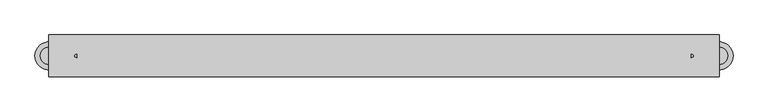
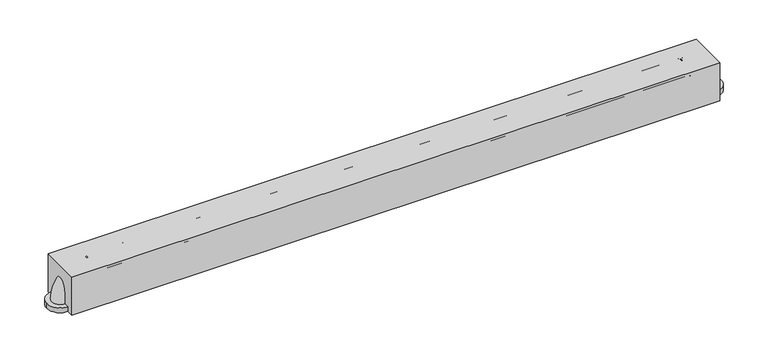
"""IFC4 building model written with IfcOpenShell, lengths in millimetres: proxy geometry, A5109 - Grab Bar, 1.25 in Dia, SS, 2 Wall, W-C Accessible : A5109 - Grab Bar, 1.25 in Dia, SS, 2 Wall, W-C Accessible."""

from ifc_helpers import new_model, si_unit, point, frame, frame_2d, origin, origin_with_axes, place, context, project, spatial, polyline, circle_curve, ellipse_curve, trimmed, segment, composite_curve, outline, extrude, source, transform, mapped, element, save
from ifc_brep_helpers import plane_surface, revolved_surface, advanced_brep


def specialty_equipment_c5804665(model_context):
    return source(origin(), model_context, "Body", "SolidModel", [
        advanced_brep(
        [(558.8, 15.875, 60.325), (558.8, -15.875, 60.325), (609.6, 15.875, 9.525), (609.6, -15.875, 9.525)],
        [
            (0, 1, circle_curve(frame((558.8, 0.0, 60.325), z_axis=(-1.0, 0.0, 0.0), x_axis=(0.0, -1.0, 0.0)), 15.875)),
            (1, 0, circle_curve(frame((558.8, 0.0, 60.325), z_axis=(-1.0, 0.0, 0.0), x_axis=(0.0, -1.0, 0.0)), 15.875)),
            (2, 3, circle_curve(frame((609.6, 0.0, 9.525), z_axis=(0.0, 0.0, -1.0), x_axis=(0.0, -1.0, 0.0)), 15.875)),
            (3, 2, circle_curve(frame((609.6, 0.0, 9.525), z_axis=(0.0, 0.0, -1.0), x_axis=(0.0, -1.0, 0.0)), 15.875)),
            (2, 0, circle_curve(frame((558.8, 15.875, 9.525), z_axis=(0.0, -1.0, 0.0), x_axis=(0.0, 0.0, 1.0)), 50.8)),
            (1, 3, circle_curve(frame((558.8, -15.875, 9.525), z_axis=(0.0, 1.0, 0.0), x_axis=(0.0, 0.0, 1.0)), 50.8)),
        ],
        [
            plane_surface(frame((558.8, 0.0, 60.325), z_axis=(-1.0, 0.0, 0.0), x_axis=(0.0, -1.0, 0.0))),
            plane_surface(frame((609.6, 0.0, 9.525), z_axis=(0.0, 0.0, -1.0), x_axis=(0.0, -1.0, 0.0))),
            revolved_surface(trimmed(ellipse_curve(frame((558.8, 0.0, 60.325), z_axis=(1.0, 0.0, 0.0), x_axis=(0.0, -1.0, 0.0)), 15.875, 15.875), [point((558.8, 15.875, 60.325))], [point((558.8, -15.875, 60.325))], True, "CARTESIAN"), (558.8, 0.0, 9.525), (0.0, -1.0, 0.0)),
            revolved_surface(trimmed(ellipse_curve(frame((558.8, 0.0, 60.325), z_axis=(1.0, 0.0, 0.0), x_axis=(0.0, -1.0, 0.0)), 15.875, 15.875), [point((558.8, -15.875, 60.325))], [point((558.8, 15.875, 60.325))], True, "CARTESIAN"), (558.8, 0.0, 9.525), (0.0, -1.0, 0.0)),
        ],
        [
            (0, [[1, 2]]),
            (1, [[3, 4]]),
            (2, [[-3, 5, -2, 6]]),
            (3, [[-4, -6, -1, -5]]),
        ],
    ),
        extrude(outline(composite_curve([segment(trimmed(circle_curve(frame_2d((609.6, 0.0)), 25.4), [point((635.0, 0.0))], [point((584.2, 0.0))], False, "CARTESIAN"), True, "CONTINUOUS"), segment(trimmed(circle_curve(frame_2d((609.6, 0.0)), 25.4), [point((584.2, 0.0))], [point((635.0, 0.0))], False, "CARTESIAN"), True, "CONTINUOUS")], self_intersect=False)), origin_with_axes(), (0.0, 0.0, 1.0), 9.525),
        advanced_brep(
        [(-558.8, 15.875, 60.325), (-558.8, -15.875, 60.325), (-609.6, 15.875, 9.525), (-609.6, -15.875, 9.525)],
        [
            (0, 1, circle_curve(frame((-558.8, 0.0, 60.325), z_axis=(1.0, 0.0, 0.0), x_axis=(0.0, -1.0, 0.0)), 15.875)),
            (1, 0, circle_curve(frame((-558.8, 0.0, 60.325), z_axis=(1.0, 0.0, 0.0), x_axis=(0.0, -1.0, 0.0)), 15.875)),
            (2, 3, circle_curve(frame((-609.6, 0.0, 9.525), z_axis=(0.0, 0.0, -1.0), x_axis=(0.0, -1.0, 0.0)), 15.875)),
            (3, 2, circle_curve(frame((-609.6, 0.0, 9.525), z_axis=(0.0, 0.0, -1.0), x_axis=(0.0, -1.0, 0.0)), 15.875)),
            (3, 1, circle_curve(frame((-558.8, -15.875, 9.525), z_axis=(0.0, 1.0, 0.0), x_axis=(0.0, 0.0, 1.0)), 50.8)),
            (0, 2, circle_curve(frame((-558.8, 15.875, 9.525), z_axis=(0.0, -1.0, 0.0), x_axis=(0.0, 0.0, 1.0)), 50.8)),
        ],
        [
            plane_surface(frame((-558.8, 0.0, 60.325), z_axis=(1.0, 0.0, 0.0), x_axis=(0.0, -1.0, 0.0))),
            plane_surface(frame((-609.6, 0.0, 9.525), z_axis=(0.0, 0.0, -1.0), x_axis=(0.0, -1.0, 0.0))),
            revolved_surface(trimmed(ellipse_curve(frame((-558.8, 0.0, 60.325), z_axis=(1.0, 0.0, 0.0), x_axis=(0.0, -1.0, 0.0)), 15.875, 15.875), [point((-558.8, 15.875, 60.325))], [point((-558.8, -15.875, 60.325))], True, "CARTESIAN"), (-558.8, 0.0, 9.525), (0.0, -1.0, 0.0)),
            revolved_surface(trimmed(ellipse_curve(frame((-558.8, 0.0, 60.325), z_axis=(1.0, 0.0, 0.0), x_axis=(0.0, -1.0, 0.0)), 15.875, 15.875), [point((-558.8, -15.875, 60.325))], [point((-558.8, 15.875, 60.325))], True, "CARTESIAN"), (-558.8, 0.0, 9.525), (0.0, -1.0, 0.0)),
        ],
        [
            (0, [[1, 2]]),
            (1, [[3, 4]]),
            (2, [[5, -1, 6, -4]]),
            (3, [[-6, -2, -5, -3]]),
        ],
    ),
        extrude(outline(composite_curve([segment(trimmed(circle_curve(frame_2d((-609.6, 0.0)), 25.4), [point((-635.0, 0.0))], [point((-584.2, 0.0))], False, "CARTESIAN"), True, "CONTINUOUS"), segment(trimmed(circle_curve(frame_2d((-609.6, 0.0)), 25.4), [point((-584.2, 0.0))], [point((-635.0, 0.0))], False, "CARTESIAN"), True, "CONTINUOUS")], self_intersect=False)), origin_with_axes(), (0.0, 0.0, 1.0), 9.525),
        extrude(outline(polyline([(609.6, -38.1), (-609.6, -38.1), (-609.6, 38.1), (609.6, 38.1), (609.6, -38.1)])), origin_with_axes(), (0.0, 0.0, 1.0), 76.2),
        extrude(outline(composite_curve([segment(trimmed(circle_curve(frame_2d((0.0, 60.325)), 15.875), [point((-15.875, 60.325))], [point((15.875, 60.325))], False, "CARTESIAN"), True, "CONTINUOUS"), segment(trimmed(circle_curve(frame_2d((0.0, 60.325)), 15.875), [point((15.875, 60.325))], [point((-15.875, 60.325))], False, "CARTESIAN"), True, "CONTINUOUS")], self_intersect=False)), frame((-558.8, 0.0, 0.0), z_axis=(1.0, 0.0, 0.0), x_axis=(0.0, 1.0, 0.0)), (0.0, 0.0, 1.0), 1117.6),
    ])


if __name__ == "__main__":
    model = new_model("IFC4")
    model_context = context("Model", 3, world=origin())
    ifc_project = project(units=[si_unit("LENGTHUNIT", "METRE", prefix="MILLI")], contexts=[model_context])
    site = spatial("IfcSite", under=ifc_project)
    building = spatial("IfcBuilding", under=site)
    placement = place(None, origin())
    specialty_equipment_shape = specialty_equipment_c5804665(model_context)
    element("IfcBuildingElementProxy", 1, Name="A5109 - Grab Bar, 1.25 in Dia, SS, 2 Wall, W-C Accessible : A5109 - Grab Bar, 1.25 in Dia, SS, 2 Wall, W-C Accessible", ObjectType="A5109 - Grab Bar, 1.25 in Dia, SS, 2 Wall, W-C Accessible : A5109 - Grab Bar, 1.25 in Dia, SS, 2 Wall, W-C Accessible", at=placement, inside=building, context=model_context, shape_type="MappedRepresentation", body=[
        mapped(specialty_equipment_shape, transform((0.0, 0.0, 0.0), x_axis=(1.0, 0.0, 0.0), y_axis=(0.0, 1.0, 0.0), z_axis=(0.0, 0.0, 1.0))),
    ])
    save(model, "model.ifc")

# Revit data of these elements
# Type "A5109 - Grab Bar, 1.25 in Dia, SS, 2 Wall, W-C Accessible : A5109 - Grab Bar, 1.25 in Dia, SS, 2 Wall, W-C Accessible"
#   Watts2 = "0"
#   Watts1 = "0"
#   Unit_Issue = "EA"
#   UTIL_6_Misc = "-"
#   UTIL_5_NonMedGas = "-"
#   UTIL_4_MiscGas = "-"
#   UTIL_3_MedGas = "-"
#   UTIL_2_Elec = "-"
#   UTIL_1_WaterDrain = "-"
#   Nomenclature = "Grab Bar, 1-1/4\" Dia., SS, 2 Wall, W/C Accessible"
#   NSN = "6530"
#   Location [instance default] = ""
#   JSN = "A5109"
#   Fund_Source_VA = "-"
#   Fund_Source_Navy = "-"
#   Fund_Source_Army = "-"
#   Fund_Source_AF = "-"
#   ELEC_Volts2 = "0"
#   ELEC_Volts1 = "0"
#   ELEC_Phase2 = "0"
#   ELEC_Phase1 = "0"
#   ELEC_HertzSwitch = "0"
#   ELEC_HertzDependent = "0"
#   ELEC_Hertz = "0"
#   ELEC_Amps2 = "0"
#   ELEC_Amps1 = "0"
#   DetailDescription = "A 1-1/4\" diameter, satin finish stainless steel, peened gripping surface, 2 wall toilet stall/ room, grab bar with concealed mounting flanges.  Snap over flanges are provided to conceal mounting screws. A selection of mounting kits and concealed anchor devices are available from the manufacturers for different types of installations. Grab bar shall comply with barrier-free accessibility guidelines for structural strength. For typical water closet applications in toilet stalls and rooms where ADA (American''s With Disabilities Act) requirements must be met."
#   CAT_VA = "A"
#   CAT_Navy = "A"
#   CAT_IHS = "-"
#   CAT_Army = "A"
#   CAT_AF = "A"
#   BTUperhour = "0"
#   Weight_IP = 7
#   Default Elevation = 2' - 9"
#   DIM_Width_IP = 4' - 9"
#   DIM_Height_IP = 0' - 3"
#   DIM_Depth_IP = 0' - 3"
#   CustomLength [instance default] = 2' - 0"
# Element 1 (IfcBuildingElementProxy, "A5109 - Grab Bar, 1.25 in Dia, SS, 2 Wall, W-C Accessible : A5109 - Grab Bar, 1.25 in Dia, SS, 2 Wall, W-C Accessible")
#   Location = "TLTU1"
#   CustomLength = 4' - 0"
#   Materials on its faces: "EquipSpace"
# Materials
#   "EquipSpace": class "Unassigned", colour RGB 221 217 195, transparency 0.5
